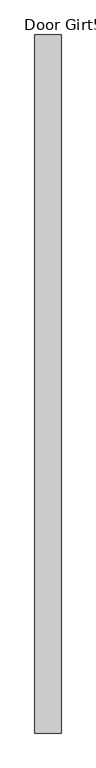
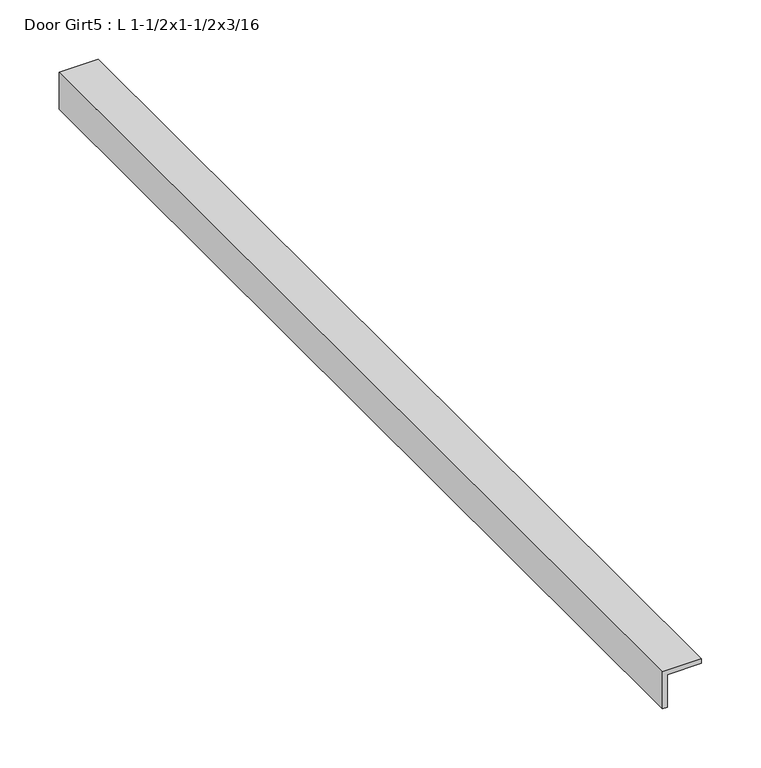
"""IFC4 building model written with IfcOpenShell, lengths in millimetres: proxy geometry, Door Girt5 : L 1-1/2x1-1/2x3/16."""

import ifcopenshell
import ifcopenshell.guid

model = None  # the IFC model being written
_history = None  # IfcOwnerHistory: only IFC2X3 demands one
_inside = {}  # id of a spatial element -> (the spatial element, [elements in it])
_under = {}  # id of a project, library or spatial element -> (it, [spatial elements below it])
_declared = {}  # id of a project -> (the project, [libraries it declares])
_typed = {}  # id of a type object -> (the type object, [elements of that type])
_made_of = {}  # id of a material, layer set ... -> (it, [elements and type objects made of it])


def new_model(schema):
    """Start an empty IFC model of exactly this schema.

    Asked for "IFC4X3", IfcOpenShell would pick the latest addendum, in which some entities
    have other attributes; the version numbers below select the first issue.
    IFC2X3 requires an IfcOwnerHistory on every rooted entity: one is made here for all.
    """
    global model, _history
    if schema == "IFC4X3":
        model = ifcopenshell.file(schema_version=(4, 3, 0, 0))
    else:
        model = ifcopenshell.file(schema=schema)
    _inside.clear()
    _under.clear()
    _declared.clear()
    _typed.clear()
    _made_of.clear()
    _history = None
    if model.schema == "IFC2X3":
        org = make("IfcOrganization", Name="unknown")
        user = make(
            "IfcPersonAndOrganization",
            ThePerson=make("IfcPerson", FamilyName="unknown"),
            TheOrganization=org,
        )
        app = make(
            "IfcApplication",
            ApplicationDeveloper=org,
            Version="unknown",
            ApplicationFullName="unknown",
            ApplicationIdentifier="unknown",
        )
        _history = make(
            "IfcOwnerHistory",
            OwningUser=user,
            OwningApplication=app,
            ChangeAction="ADDED",
            CreationDate=0,
        )
    return model


def make(cls, **values):
    """One entity of the class cls with the attributes given. An attribute that is None is left unset."""
    return model.create_entity(
        cls, **{name: value for name, value in values.items() if value is not None}
    )


def rooted(cls, **values):
    """An entity with a GlobalId (a new one), such as an element, a storey or a relation."""
    return make(cls, GlobalId=ifcopenshell.guid.new(), OwnerHistory=_history, **values)


def si_unit(unit_type, name, prefix=None):
    """IfcSIUnit, for example si_unit("LENGTHUNIT", "METRE", prefix="MILLI")."""
    return make("IfcSIUnit", UnitType=unit_type, Prefix=prefix, Name=name)


def assignment(units):
    """IfcUnitAssignment: the units of a project."""
    return None if units is None else make("IfcUnitAssignment", Units=units)


def point(xyz):
    """IfcCartesianPoint."""
    return None if xyz is None else make("IfcCartesianPoint", Coordinates=xyz)


def direction(xyz):
    """IfcDirection."""
    return None if xyz is None else make("IfcDirection", DirectionRatios=xyz)


def frame(location, z_axis=None, x_axis=None):
    """IfcAxis2Placement3D, a coordinate frame: its origin and axes. An axis left out is left unset."""
    return make(
        "IfcAxis2Placement3D",
        Location=point(location),
        Axis=direction(z_axis),
        RefDirection=direction(x_axis),
    )


def origin():
    """The frame at (0, 0, 0) with its axes left unset."""
    return frame((0.0, 0.0, 0.0))


def place(relative_to, where):
    """IfcLocalPlacement: puts the frame where relative to a parent placement (None: the world)."""
    return make(
        "IfcLocalPlacement", PlacementRelTo=relative_to, RelativePlacement=where
    )


def context(
    kind, dimensions, precision=None, world=None, true_north=None, identifier=None
):
    """IfcGeometricRepresentationContext, for example the 3D "Model" context."""
    return make(
        "IfcGeometricRepresentationContext",
        ContextIdentifier=identifier,
        ContextType=kind,
        CoordinateSpaceDimension=dimensions,
        Precision=precision,
        WorldCoordinateSystem=world,
        TrueNorth=true_north,
    )


def project(units=None, contexts=None):
    """IfcProject with its units and contexts."""
    return rooted(
        "IfcProject",
        Name="project",
        RepresentationContexts=contexts,
        UnitsInContext=assignment(units),
    )


def spatial(cls, under=None, at=None, **own):
    """A site, building, storey or space (cls), placed at a placement, below another one or the project."""
    s = rooted(cls, ObjectPlacement=at, **own)
    if under is not None:
        _under.setdefault(under.id(), (under, []))[1].append(s)
    return s


def polyline(points):
    """IfcPolyline through the points."""
    return make("IfcPolyline", Points=[point(p) for p in points])


def outline(outer, holes=None, kind="AREA"):
    """IfcArbitraryClosedProfileDef: a profile drawn as a closed curve; with holes, ...WithVoids."""
    if holes is None:
        return make("IfcArbitraryClosedProfileDef", ProfileType=kind, OuterCurve=outer)
    return make(
        "IfcArbitraryProfileDefWithVoids",
        ProfileType=kind,
        OuterCurve=outer,
        InnerCurves=holes,
    )


def extrude(swept, where, along, depth):
    """IfcExtrudedAreaSolid: the profile swept, set in the frame where, extruded along a direction by depth."""
    return make(
        "IfcExtrudedAreaSolid",
        SweptArea=swept,
        Position=where,
        ExtrudedDirection=direction(along),
        Depth=depth,
    )


def shape(context_of_items, identifier, shape_type, items):
    """IfcShapeRepresentation: the items that make up one representation, for example the "Body"."""
    return make(
        "IfcShapeRepresentation",
        ContextOfItems=context_of_items,
        RepresentationIdentifier=identifier,
        RepresentationType=shape_type,
        Items=items,
    )


def source(mapping_origin, context_of_items, identifier, shape_type, items):
    """IfcRepresentationMap: a shape defined once, which mapped items show again and again."""
    return make(
        "IfcRepresentationMap",
        MappingOrigin=mapping_origin,
        MappedRepresentation=shape(context_of_items, identifier, shape_type, items),
    )


def transform(
    local_origin,
    x_axis=None,
    y_axis=None,
    z_axis=None,
    scale=None,
    scale2=None,
    scale3=None,
    uniform=True,
):
    """IfcCartesianTransformationOperator3D, or its non-uniform kind. x_axis, y_axis, z_axis: its Axis1, 2, 3."""
    if uniform:
        return make(
            "IfcCartesianTransformationOperator3D",
            Axis1=direction(x_axis),
            Axis2=direction(y_axis),
            LocalOrigin=point(local_origin),
            Scale=scale,
            Axis3=direction(z_axis),
        )
    return make(
        "IfcCartesianTransformationOperator3DnonUniform",
        Axis1=direction(x_axis),
        Axis2=direction(y_axis),
        LocalOrigin=point(local_origin),
        Scale=scale,
        Axis3=direction(z_axis),
        Scale2=scale2,
        Scale3=scale3,
    )


def mapped(mapping_source, mapping_target):
    """IfcMappedItem: shows the shape of a source again, moved by a transform."""
    return make(
        "IfcMappedItem", MappingSource=mapping_source, MappingTarget=mapping_target
    )


def made_of(thing, what):
    """Note that an element or type object is made of a material, layer set ...; save() writes the relation."""
    if what is not None:
        _made_of.setdefault(what.id(), (what, []))[1].append(thing)
    return thing


def element(
    cls,
    number,
    at=None,
    inside=None,
    cuts=None,
    type_object=None,
    material=None,
    context=None,
    identifier="Body",
    shape_type=None,
    held_by="IfcProductDefinitionShape",
    body=None,
    shapes=None,
    **own,
):
    """One element of the class cls, such as IfcWall. Its Tag is "e" and its number.

    at: its placement. inside: the storey or other place that contains it. cuts: it is an
    opening in that element (IfcRelVoidsElement). A single representation is given by context,
    identifier, shape_type and body (its items); several are given by shapes. held_by: the class
    of the entity that holds the representations. save() writes the other relations.
    """
    e = rooted(cls, Tag="e%d" % number, ObjectPlacement=at, **own)
    if body is not None:
        shapes = [shape(context, identifier, shape_type, body)]
    if shapes is not None:
        e.Representation = make(held_by, Representations=shapes)
    if inside is not None:
        _inside.setdefault(inside.id(), (inside, []))[1].append(e)
    if cuts is not None:
        rooted(
            "IfcRelVoidsElement", RelatingBuildingElement=cuts, RelatedOpeningElement=e
        )
    if type_object is not None:
        _typed.setdefault(type_object.id(), (type_object, []))[1].append(e)
    return made_of(e, material)


def aggregate(whole, parts):
    """IfcRelAggregates: a whole, such as a stair, and the parts it consists of."""
    return rooted("IfcRelAggregates", RelatingObject=whole, RelatedObjects=parts)


def save(model, path):
    """Write the relations noted so far, then the file.

    IfcRelAggregates (storeys below a building ...), IfcRelContainedInSpatialStructure (elements
    in a storey), IfcRelDefinesByType, IfcRelAssociatesMaterial and IfcRelDeclares: one each for
    every whole, place, type object, material and project.
    """
    for whole, parts in _under.values():
        aggregate(whole, parts)
    for where, things in _inside.values():
        rooted(
            "IfcRelContainedInSpatialStructure",
            RelatedElements=things,
            RelatingStructure=where,
        )
    for kind, things in _typed.values():
        rooted("IfcRelDefinesByType", RelatedObjects=things, RelatingType=kind)
    for what, things in _made_of.values():
        rooted("IfcRelAssociatesMaterial", RelatedObjects=things, RelatingMaterial=what)
    for by, libraries in _declared.values():
        rooted("IfcRelDeclares", RelatingContext=by, RelatedDefinitions=libraries)
    model.write(path)


def door_girt5_l_1_1_2x1_1_2x3_16_e85b96be(model_context):
    return source(origin(), model_context, "Body", "SweptSolid", [
        extrude(outline(polyline([(1625.6, 587403.9934739), (1625.6, 587365.8934739), (1587.5, 587365.8934739), (1587.5, 587370.6559739), (1620.8375, 587370.6559739), (1620.8375, 587403.9934739), (1625.6, 587403.9934739)])), frame((0.0, -532839.3663841, 0.0), z_axis=(0.0, 1.0, 0.0), x_axis=(0.0, 0.0, 1.0)), (0.0, 0.0, 1.0), 1017.5875),
    ])


if __name__ == "__main__":
    model = new_model("IFC4")
    model_context = context("Model", 3, world=origin())
    ifc_project = project(units=[si_unit("LENGTHUNIT", "METRE", prefix="MILLI")], contexts=[model_context])
    site = spatial("IfcSite", under=ifc_project)
    building = spatial("IfcBuilding", under=site)
    placement = place(None, origin())
    door_girt5_l_1_1_2x1_1_2x3_16_shape = door_girt5_l_1_1_2x1_1_2x3_16_e85b96be(model_context)
    element("IfcBuildingElementProxy", 1, Name="Door Girt5 : L 1-1/2x1-1/2x3/16", ObjectType="Door Girt5 : L 1-1/2x1-1/2x3/16", at=placement, inside=building, context=model_context, shape_type="MappedRepresentation", body=[
        mapped(door_girt5_l_1_1_2x1_1_2x3_16_shape, transform((0.0, 0.0, 0.0), x_axis=(1.0, 0.0, 0.0), y_axis=(0.0, 1.0, 0.0), z_axis=(0.0, 0.0, 1.0))),
    ])
    save(model, "model.ifc")

# Revit data of these elements
# Element 1 (IfcBuildingElementProxy, "Door Girt5 : L 1-1/2x1-1/2x3/16")
#   Materials on its faces: "1-1/2\"X1-1/2\" GALV. STL L"
# Materials
#   "1-1/2\"X1-1/2\" GALV. STL L": class "Generic", colour RGB 211 211 207, transparency 0, Cost = 0
